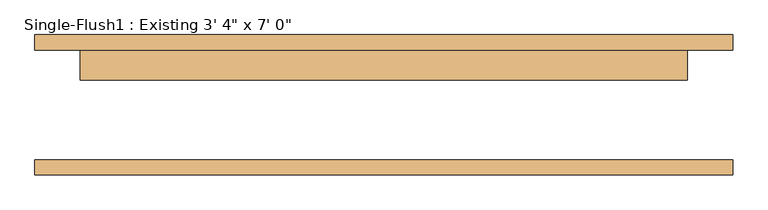
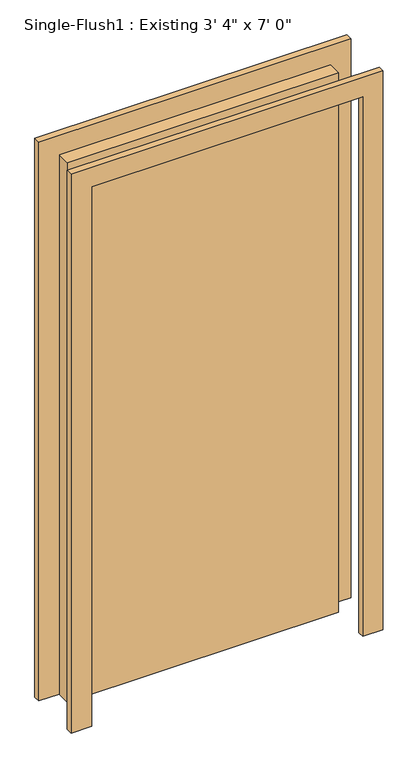
"""IFC4 building model written with IfcOpenShell, lengths in millimetres: door geometry."""

from ifc_helpers import new_model, si_unit, frame, origin, origin_with_axes, place, context, project, spatial, polyline, outline, extrude, source, transform, mapped, element, save


def door_bd3f6991(model_context):
    return source(origin(), model_context, "Body", "SweptSolid", [
        extrude(outline(polyline([(2209.8, -584.2), (0.0, -584.2), (0.0, -508.0), (2133.6, -508.0), (2133.6, 508.0), (0.0, 508.0), (0.0, 584.2), (2209.8, 584.2), (2209.8, -584.2)])), frame((0.0, 92.075, 0.0), z_axis=(0.0, 1.0, 0.0), x_axis=(0.0, 0.0, 1.0)), (0.0, 0.0, 1.0), 25.4),
        extrude(outline(polyline([(2209.8, 584.2), (2209.8, -584.2), (0.0, -584.2), (0.0, -508.0), (2133.6, -508.0), (2133.6, 508.0), (0.0, 508.0), (0.0, 584.2), (2209.8, 584.2)])), frame((0.0, -117.475, 0.0), z_axis=(0.0, 1.0, 0.0), x_axis=(0.0, 0.0, 1.0)), (0.0, 0.0, 1.0), 25.4),
        extrude(outline(polyline([(508.0, 41.275), (-508.0, 41.275), (-508.0, 92.075), (508.0, 92.075), (508.0, 41.275)])), origin_with_axes(), (0.0, 0.0, 1.0), 2133.6),
    ])


if __name__ == "__main__":
    model = new_model("IFC4")
    model_context = context("Model", 3, world=origin())
    ifc_project = project(units=[si_unit("LENGTHUNIT", "METRE", prefix="MILLI")], contexts=[model_context])
    site = spatial("IfcSite", under=ifc_project)
    building = spatial("IfcBuilding", under=site)
    placement = place(None, origin())
    door_shape = door_bd3f6991(model_context)
    element("IfcDoor", 1, ObjectType="Single-Flush1 : Existing 3' 4\" x 7' 0\"", at=placement, inside=building, context=model_context, shape_type="MappedRepresentation", body=[
        mapped(door_shape, transform((0.0, 0.0, 0.0), x_axis=(1.0, 0.0, 0.0), y_axis=(0.0, 1.0, 0.0), z_axis=(0.0, 0.0, 1.0))),
    ])
    save(model, "model.ifc")

# Revit data of these elements
# Type "Single-Flush1 : Existing 3' 4\" x 7' 0\""
#   Type Mark = "EX"
#   Construction Type Id = "MDOOR"
#   Assembly Code = "C1020"
#   Analytic Construction = "Metal"
#   Thickness = 0' - 2"
#   Heat Transfer Coefficient (U) = 3.7021 W/(m²·K)
#   Height = 7' - 0"
#   Trim Projection Ext = 0' - 1"
#   Trim Projection Int = 0' - 1"
#   Trim Width = 0' - 3"
#   Width = 3' - 4"
#   Door Material = Door - Panel
#   Frame Material = Door - Frame
#   Visual Light Transmittance = 0
#   Solar Heat Gain Coefficient = 0
#   Function = (empty or 0)
#   Wall Closure = (empty or 0)
# Element 1 (IfcDoor, "Single-Flush1 : Existing 3' 4\" x 7' 0\"")
#   Materials on its faces: "Door - Frame", "Door - Panel"
# Materials
#   "Door - Panel": class "Wood", colour RGB 255 255 255, transparency 0, Cost = 0
#   "Door - Frame": class "Miscellaneous", colour RGB 255 255 255, transparency 0, Cost = 0
